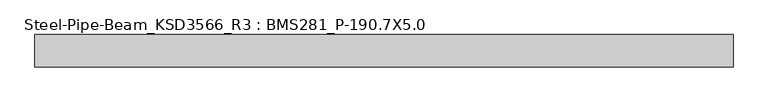
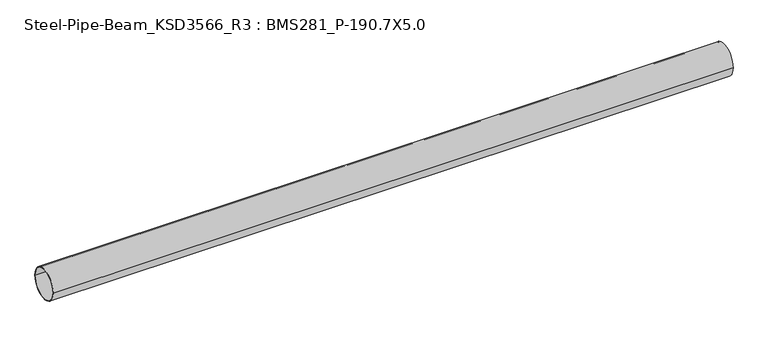
"""IFC4 building model written with IfcOpenShell, lengths in millimetres: member geometry, Steel-Pipe-Beam_KSD3566_R3 : BMS281_P-190.7X5.0."""

from ifc_helpers import new_model, si_unit, point, frame, origin, origin_2d, place, context, project, spatial, circle_curve, trimmed, segment, composite_curve, outline, extrude, source, transform, mapped, element, save


def steel_pipe_beam_ksd3566_r3_bms281_p_190_7x5_0_432b37f6(model_context):
    return source(origin(), model_context, "Body", "SweptSolid", [
        extrude(outline(composite_curve([segment(trimmed(circle_curve(origin_2d(), 95.35), [point((95.35, 0.0))], [point((-95.35, 0.0))], False, "CARTESIAN"), True, "CONTINUOUS"), segment(trimmed(circle_curve(origin_2d(), 95.35), [point((-95.35, 0.0))], [point((95.35, 0.0))], False, "CARTESIAN"), True, "CONTINUOUS")], self_intersect=False), holes=[composite_curve([segment(trimmed(circle_curve(origin_2d(), 90.35), [point((-90.35, 0.0))], [point((90.35, 0.0))], True, "CARTESIAN"), True, "CONTINUOUS"), segment(trimmed(circle_curve(origin_2d(), 90.35), [point((90.35, 0.0))], [point((-90.35, 0.0))], True, "CARTESIAN"), True, "CONTINUOUS")], self_intersect=False)]), frame((-2059.528929, 0.0, 0.0), z_axis=(1.0, 0.0, 0.0), x_axis=(0.0, 1.0, 0.0)), (0.0, 0.0, 1.0), 4105.6761578),
    ])


if __name__ == "__main__":
    model = new_model("IFC4")
    model_context = context("Model", 3, world=origin())
    ifc_project = project(units=[si_unit("LENGTHUNIT", "METRE", prefix="MILLI")], contexts=[model_context])
    site = spatial("IfcSite", under=ifc_project)
    building = spatial("IfcBuilding", under=site)
    placement = place(None, origin())
    steel_pipe_beam_ksd3566_r3_bms281_p_190_7x5_0_shape = steel_pipe_beam_ksd3566_r3_bms281_p_190_7x5_0_432b37f6(model_context)
    element("IfcMember", 1, ObjectType="Steel-Pipe-Beam_KSD3566_R3 : BMS281_P-190.7X5.0", at=placement, inside=building, context=model_context, shape_type="MappedRepresentation", body=[
        mapped(steel_pipe_beam_ksd3566_r3_bms281_p_190_7x5_0_shape, transform((0.0, 0.0, 0.0), x_axis=(1.0, 0.0, 0.0), y_axis=(0.0, 1.0, 0.0), z_axis=(0.0, 0.0, 1.0))),
    ])
    save(model, "model.ifc")

# Revit data of these elements
# Type "Steel-Pipe-Beam_KSD3566_R3 : BMS281_P-190.7X5.0"
#   Keynote = "P-190.7X5.0"
#   SteelWeight = "Light"
#   t = 0.0050 m
#   Surface Area = 0.599102 m²/m
#   Section Area = 29.1697 cm²
#   Mass per Unit Length = 22.8982 kg/m
#   Length [instance default] = 1.5000 m
#   D = 0.1907 m
#   hec_material4 [instance default] = none
#   hec_material3 [instance default] = none
#   hec_material2 [instance default] = none
#   hec_material1 [instance default] = none
#   Structural Material [instance default] = Steel, 45-345
#   Assembly Code = ""
# Element 1 (IfcMember, "Steel-Pipe-Beam_KSD3566_R3 : BMS281_P-190.7X5.0")
#   Structural Material = none
# Materials
#   "Steel, 45-345": class "Metal", colour RGB 189 187 185, transparency 0, Description = "Steel 345 MPa", Cost = 0
